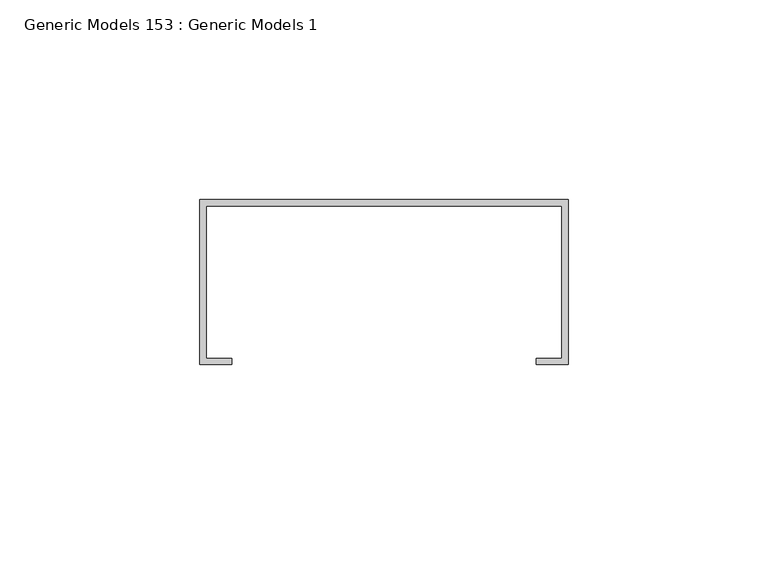
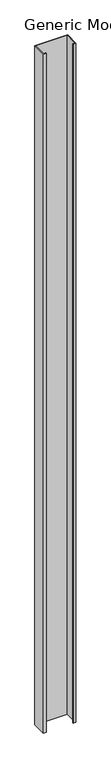
"""IFC4 building model written with IfcOpenShell, lengths in millimetres: proxy geometry, Generic Models 153 : Generic Models 1."""

from ifc_helpers import new_model, si_unit, frame, origin, place, context, project, spatial, polyline, outline, extrude, source, transform, mapped, element, save


def generic_models_153_generic_models_1_113e5eee(model_context):
    return source(origin(), model_context, "Body", "SweptSolid", [
        extrude(outline(polyline([(51003.2, 630.2375), (51003.2, 588.9625), (50995.2625, 588.9625), (50995.2625, 590.55), (51001.6125, 590.55), (51001.6125, 628.65), (50912.7125, 628.65), (50912.7125, 590.55), (50919.0625, 590.55), (50919.0625, 588.9625), (50911.125, 588.9625), (50911.125, 630.2375), (51003.2, 630.2375)])), frame((0.0, 0.0, 1.5875), z_axis=(0.0, 0.0, 1.0), x_axis=(1.0, 0.0, 0.0)), (0.0, 0.0, 1.0), 2025.65),
    ])


if __name__ == "__main__":
    model = new_model("IFC4")
    model_context = context("Model", 3, world=origin())
    ifc_project = project(units=[si_unit("LENGTHUNIT", "METRE", prefix="MILLI")], contexts=[model_context])
    site = spatial("IfcSite", under=ifc_project)
    building = spatial("IfcBuilding", under=site)
    placement = place(None, origin())
    generic_models_153_generic_models_1_shape = generic_models_153_generic_models_1_113e5eee(model_context)
    element("IfcBuildingElementProxy", 1, Name="Generic Models 153 : Generic Models 1", ObjectType="Generic Models 153 : Generic Models 1", at=placement, inside=building, context=model_context, shape_type="MappedRepresentation", body=[
        mapped(generic_models_153_generic_models_1_shape, transform((0.0, 0.0, 0.0), x_axis=(1.0, 0.0, 0.0), y_axis=(0.0, 1.0, 0.0), z_axis=(0.0, 0.0, 1.0))),
    ])
    save(model, "model.ifc")

# Revit data of these elements
# Element 1 (IfcBuildingElementProxy, "Generic Models 153 : Generic Models 1")
#   Materials on its faces: "EXISTING STUDS"
# Materials
#   "EXISTING STUDS": class "Unassigned", colour RGB 210 209 208, transparency 0, Keynote = "M05121300.02", Cost = 0
